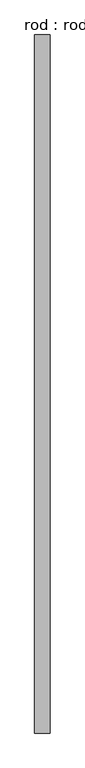
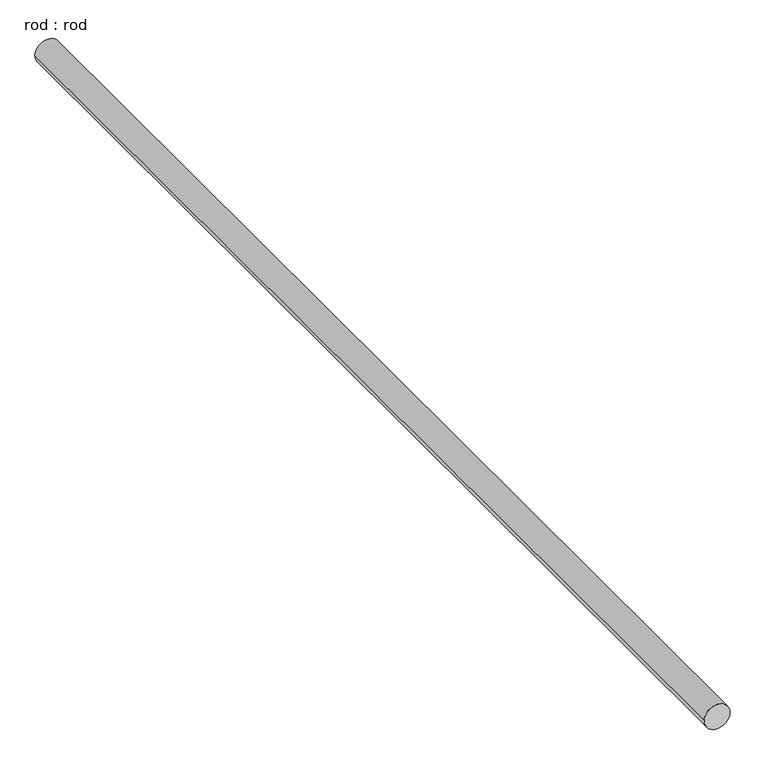
"""IFC4 building model written with IfcOpenShell, lengths in millimetres: proxy geometry, rod : rod."""

import ifcopenshell
import ifcopenshell.guid

model = None  # the IFC model being written
_history = None  # IfcOwnerHistory: only IFC2X3 demands one
_inside = {}  # id of a spatial element -> (the spatial element, [elements in it])
_under = {}  # id of a project, library or spatial element -> (it, [spatial elements below it])
_declared = {}  # id of a project -> (the project, [libraries it declares])
_typed = {}  # id of a type object -> (the type object, [elements of that type])
_made_of = {}  # id of a material, layer set ... -> (it, [elements and type objects made of it])


def new_model(schema):
    """Start an empty IFC model of exactly this schema.

    Asked for "IFC4X3", IfcOpenShell would pick the latest addendum, in which some entities
    have other attributes; the version numbers below select the first issue.
    IFC2X3 requires an IfcOwnerHistory on every rooted entity: one is made here for all.
    """
    global model, _history
    if schema == "IFC4X3":
        model = ifcopenshell.file(schema_version=(4, 3, 0, 0))
    else:
        model = ifcopenshell.file(schema=schema)
    _inside.clear()
    _under.clear()
    _declared.clear()
    _typed.clear()
    _made_of.clear()
    _history = None
    if model.schema == "IFC2X3":
        org = make("IfcOrganization", Name="unknown")
        user = make(
            "IfcPersonAndOrganization",
            ThePerson=make("IfcPerson", FamilyName="unknown"),
            TheOrganization=org,
        )
        app = make(
            "IfcApplication",
            ApplicationDeveloper=org,
            Version="unknown",
            ApplicationFullName="unknown",
            ApplicationIdentifier="unknown",
        )
        _history = make(
            "IfcOwnerHistory",
            OwningUser=user,
            OwningApplication=app,
            ChangeAction="ADDED",
            CreationDate=0,
        )
    return model


def make(cls, **values):
    """One entity of the class cls with the attributes given. An attribute that is None is left unset."""
    return model.create_entity(
        cls, **{name: value for name, value in values.items() if value is not None}
    )


def rooted(cls, **values):
    """An entity with a GlobalId (a new one), such as an element, a storey or a relation."""
    return make(cls, GlobalId=ifcopenshell.guid.new(), OwnerHistory=_history, **values)


def si_unit(unit_type, name, prefix=None):
    """IfcSIUnit, for example si_unit("LENGTHUNIT", "METRE", prefix="MILLI")."""
    return make("IfcSIUnit", UnitType=unit_type, Prefix=prefix, Name=name)


def assignment(units):
    """IfcUnitAssignment: the units of a project."""
    return None if units is None else make("IfcUnitAssignment", Units=units)


def point(xyz):
    """IfcCartesianPoint."""
    return None if xyz is None else make("IfcCartesianPoint", Coordinates=xyz)


def direction(xyz):
    """IfcDirection."""
    return None if xyz is None else make("IfcDirection", DirectionRatios=xyz)


def frame(location, z_axis=None, x_axis=None):
    """IfcAxis2Placement3D, a coordinate frame: its origin and axes. An axis left out is left unset."""
    return make(
        "IfcAxis2Placement3D",
        Location=point(location),
        Axis=direction(z_axis),
        RefDirection=direction(x_axis),
    )


def frame_2d(location, x_axis=None):
    """IfcAxis2Placement2D, a coordinate frame in the plane: its origin and x axis."""
    return make(
        "IfcAxis2Placement2D", Location=point(location), RefDirection=direction(x_axis)
    )


def origin():
    """The frame at (0, 0, 0) with its axes left unset."""
    return frame((0.0, 0.0, 0.0))


def place(relative_to, where):
    """IfcLocalPlacement: puts the frame where relative to a parent placement (None: the world)."""
    return make(
        "IfcLocalPlacement", PlacementRelTo=relative_to, RelativePlacement=where
    )


def context(
    kind, dimensions, precision=None, world=None, true_north=None, identifier=None
):
    """IfcGeometricRepresentationContext, for example the 3D "Model" context."""
    return make(
        "IfcGeometricRepresentationContext",
        ContextIdentifier=identifier,
        ContextType=kind,
        CoordinateSpaceDimension=dimensions,
        Precision=precision,
        WorldCoordinateSystem=world,
        TrueNorth=true_north,
    )


def project(units=None, contexts=None):
    """IfcProject with its units and contexts."""
    return rooted(
        "IfcProject",
        Name="project",
        RepresentationContexts=contexts,
        UnitsInContext=assignment(units),
    )


def spatial(cls, under=None, at=None, **own):
    """A site, building, storey or space (cls), placed at a placement, below another one or the project."""
    s = rooted(cls, ObjectPlacement=at, **own)
    if under is not None:
        _under.setdefault(under.id(), (under, []))[1].append(s)
    return s


def circle_curve(where, radius):
    """IfcCircle in the frame where."""
    return make("IfcCircle", Position=where, Radius=radius)


def trimmed(basis, trim1, trim2, sense, master):
    """IfcTrimmedCurve: the piece of a basis curve between two trims."""
    return make(
        "IfcTrimmedCurve",
        BasisCurve=basis,
        Trim1=trim1,
        Trim2=trim2,
        SenseAgreement=sense,
        MasterRepresentation=master,
    )


def segment(curve, same_sense, transition):
    """IfcCompositeCurveSegment."""
    return make(
        "IfcCompositeCurveSegment",
        Transition=transition,
        SameSense=same_sense,
        ParentCurve=curve,
    )


def composite_curve(segments, self_intersect=None):
    """IfcCompositeCurve: segments joined end to end."""
    return make("IfcCompositeCurve", Segments=segments, SelfIntersect=self_intersect)


def outline(outer, holes=None, kind="AREA"):
    """IfcArbitraryClosedProfileDef: a profile drawn as a closed curve; with holes, ...WithVoids."""
    if holes is None:
        return make("IfcArbitraryClosedProfileDef", ProfileType=kind, OuterCurve=outer)
    return make(
        "IfcArbitraryProfileDefWithVoids",
        ProfileType=kind,
        OuterCurve=outer,
        InnerCurves=holes,
    )


def extrude(swept, where, along, depth):
    """IfcExtrudedAreaSolid: the profile swept, set in the frame where, extruded along a direction by depth."""
    return make(
        "IfcExtrudedAreaSolid",
        SweptArea=swept,
        Position=where,
        ExtrudedDirection=direction(along),
        Depth=depth,
    )


def shape(context_of_items, identifier, shape_type, items):
    """IfcShapeRepresentation: the items that make up one representation, for example the "Body"."""
    return make(
        "IfcShapeRepresentation",
        ContextOfItems=context_of_items,
        RepresentationIdentifier=identifier,
        RepresentationType=shape_type,
        Items=items,
    )


def source(mapping_origin, context_of_items, identifier, shape_type, items):
    """IfcRepresentationMap: a shape defined once, which mapped items show again and again."""
    return make(
        "IfcRepresentationMap",
        MappingOrigin=mapping_origin,
        MappedRepresentation=shape(context_of_items, identifier, shape_type, items),
    )


def transform(
    local_origin,
    x_axis=None,
    y_axis=None,
    z_axis=None,
    scale=None,
    scale2=None,
    scale3=None,
    uniform=True,
):
    """IfcCartesianTransformationOperator3D, or its non-uniform kind. x_axis, y_axis, z_axis: its Axis1, 2, 3."""
    if uniform:
        return make(
            "IfcCartesianTransformationOperator3D",
            Axis1=direction(x_axis),
            Axis2=direction(y_axis),
            LocalOrigin=point(local_origin),
            Scale=scale,
            Axis3=direction(z_axis),
        )
    return make(
        "IfcCartesianTransformationOperator3DnonUniform",
        Axis1=direction(x_axis),
        Axis2=direction(y_axis),
        LocalOrigin=point(local_origin),
        Scale=scale,
        Axis3=direction(z_axis),
        Scale2=scale2,
        Scale3=scale3,
    )


def mapped(mapping_source, mapping_target):
    """IfcMappedItem: shows the shape of a source again, moved by a transform."""
    return make(
        "IfcMappedItem", MappingSource=mapping_source, MappingTarget=mapping_target
    )


def made_of(thing, what):
    """Note that an element or type object is made of a material, layer set ...; save() writes the relation."""
    if what is not None:
        _made_of.setdefault(what.id(), (what, []))[1].append(thing)
    return thing


def element(
    cls,
    number,
    at=None,
    inside=None,
    cuts=None,
    type_object=None,
    material=None,
    context=None,
    identifier="Body",
    shape_type=None,
    held_by="IfcProductDefinitionShape",
    body=None,
    shapes=None,
    **own,
):
    """One element of the class cls, such as IfcWall. Its Tag is "e" and its number.

    at: its placement. inside: the storey or other place that contains it. cuts: it is an
    opening in that element (IfcRelVoidsElement). A single representation is given by context,
    identifier, shape_type and body (its items); several are given by shapes. held_by: the class
    of the entity that holds the representations. save() writes the other relations.
    """
    e = rooted(cls, Tag="e%d" % number, ObjectPlacement=at, **own)
    if body is not None:
        shapes = [shape(context, identifier, shape_type, body)]
    if shapes is not None:
        e.Representation = make(held_by, Representations=shapes)
    if inside is not None:
        _inside.setdefault(inside.id(), (inside, []))[1].append(e)
    if cuts is not None:
        rooted(
            "IfcRelVoidsElement", RelatingBuildingElement=cuts, RelatedOpeningElement=e
        )
    if type_object is not None:
        _typed.setdefault(type_object.id(), (type_object, []))[1].append(e)
    return made_of(e, material)


def aggregate(whole, parts):
    """IfcRelAggregates: a whole, such as a stair, and the parts it consists of."""
    return rooted("IfcRelAggregates", RelatingObject=whole, RelatedObjects=parts)


def save(model, path):
    """Write the relations noted so far, then the file.

    IfcRelAggregates (storeys below a building ...), IfcRelContainedInSpatialStructure (elements
    in a storey), IfcRelDefinesByType, IfcRelAssociatesMaterial and IfcRelDeclares: one each for
    every whole, place, type object, material and project.
    """
    for whole, parts in _under.values():
        aggregate(whole, parts)
    for where, things in _inside.values():
        rooted(
            "IfcRelContainedInSpatialStructure",
            RelatedElements=things,
            RelatingStructure=where,
        )
    for kind, things in _typed.values():
        rooted("IfcRelDefinesByType", RelatedObjects=things, RelatingType=kind)
    for what, things in _made_of.values():
        rooted("IfcRelAssociatesMaterial", RelatedObjects=things, RelatingMaterial=what)
    for by, libraries in _declared.values():
        rooted("IfcRelDeclares", RelatingContext=by, RelatedDefinitions=libraries)
    model.write(path)


def rod_rod_e7b30b47(model_context):
    return source(origin(), model_context, "Body", "SweptSolid", [
        extrude(outline(composite_curve([segment(trimmed(circle_curve(frame_2d((0.0108462, 0.0)), 200.0), [point((0.0108462, 200.0))], [point((0.0108462, -200.0))], False, "CARTESIAN"), True, "CONTINUOUS"), segment(trimmed(circle_curve(frame_2d((0.0108462, 0.0)), 200.0), [point((0.0108462, -200.0))], [point((0.0108462, 200.0))], False, "CARTESIAN"), True, "CONTINUOUS")], self_intersect=False)), frame((0.0, -4924.1391513, 0.0), z_axis=(0.0, 1.0, 0.0), x_axis=(0.0, 0.0, 1.0)), (0.0, 0.0, 1.0), 18033.7355333),
    ])


if __name__ == "__main__":
    model = new_model("IFC4")
    model_context = context("Model", 3, world=origin())
    ifc_project = project(units=[si_unit("LENGTHUNIT", "METRE", prefix="MILLI")], contexts=[model_context])
    site = spatial("IfcSite", under=ifc_project)
    building = spatial("IfcBuilding", under=site)
    placement = place(None, origin())
    rod_rod_shape = rod_rod_e7b30b47(model_context)
    element("IfcBuildingElementProxy", 1, Name="rod : rod", ObjectType="rod : rod", at=placement, inside=building, context=model_context, shape_type="MappedRepresentation", body=[
        mapped(rod_rod_shape, transform((0.0, 0.0, 0.0), x_axis=(1.0, 0.0, 0.0), y_axis=(0.0, 1.0, 0.0), z_axis=(0.0, 0.0, 1.0))),
    ])
    save(model, "model.ifc")

# Revit data of these elements
# Type "rod : rod"
#   Default Elevation = 0
